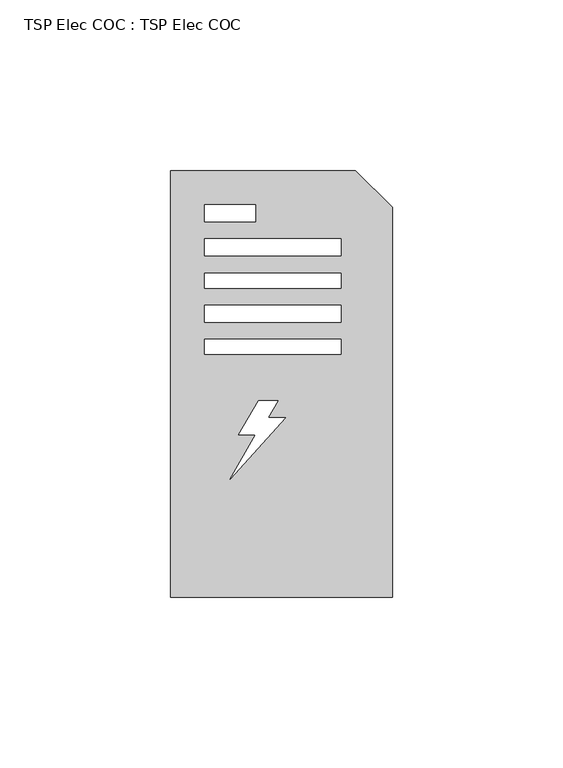
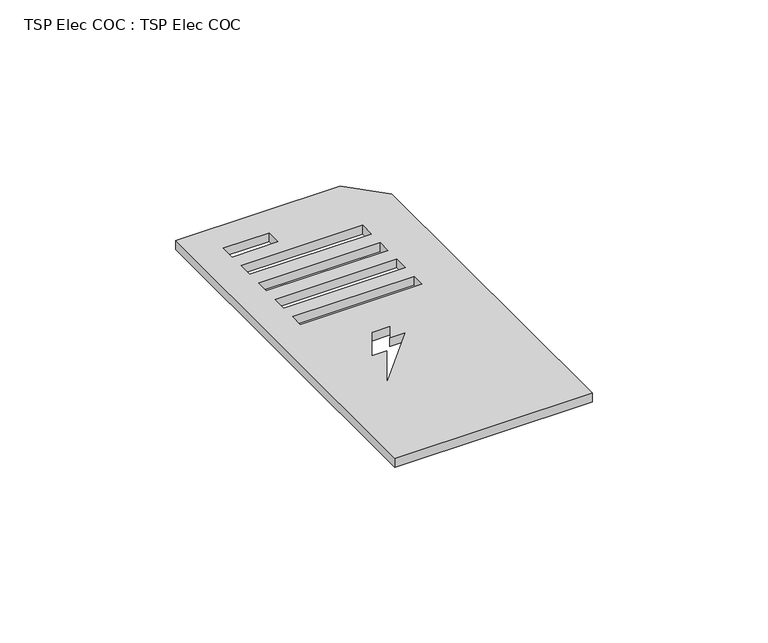
"""IFC4 building model written with IfcOpenShell, lengths in millimetres: proxy geometry, TSP Elec COC : TSP Elec COC."""

import ifcopenshell
import ifcopenshell.guid

model = None  # the IFC model being written
_history = None  # IfcOwnerHistory: only IFC2X3 demands one
_inside = {}  # id of a spatial element -> (the spatial element, [elements in it])
_under = {}  # id of a project, library or spatial element -> (it, [spatial elements below it])
_declared = {}  # id of a project -> (the project, [libraries it declares])
_typed = {}  # id of a type object -> (the type object, [elements of that type])
_made_of = {}  # id of a material, layer set ... -> (it, [elements and type objects made of it])


def new_model(schema):
    """Start an empty IFC model of exactly this schema.

    Asked for "IFC4X3", IfcOpenShell would pick the latest addendum, in which some entities
    have other attributes; the version numbers below select the first issue.
    IFC2X3 requires an IfcOwnerHistory on every rooted entity: one is made here for all.
    """
    global model, _history
    if schema == "IFC4X3":
        model = ifcopenshell.file(schema_version=(4, 3, 0, 0))
    else:
        model = ifcopenshell.file(schema=schema)
    _inside.clear()
    _under.clear()
    _declared.clear()
    _typed.clear()
    _made_of.clear()
    _history = None
    if model.schema == "IFC2X3":
        org = make("IfcOrganization", Name="unknown")
        user = make(
            "IfcPersonAndOrganization",
            ThePerson=make("IfcPerson", FamilyName="unknown"),
            TheOrganization=org,
        )
        app = make(
            "IfcApplication",
            ApplicationDeveloper=org,
            Version="unknown",
            ApplicationFullName="unknown",
            ApplicationIdentifier="unknown",
        )
        _history = make(
            "IfcOwnerHistory",
            OwningUser=user,
            OwningApplication=app,
            ChangeAction="ADDED",
            CreationDate=0,
        )
    return model


def make(cls, **values):
    """One entity of the class cls with the attributes given. An attribute that is None is left unset."""
    return model.create_entity(
        cls, **{name: value for name, value in values.items() if value is not None}
    )


def rooted(cls, **values):
    """An entity with a GlobalId (a new one), such as an element, a storey or a relation."""
    return make(cls, GlobalId=ifcopenshell.guid.new(), OwnerHistory=_history, **values)


def si_unit(unit_type, name, prefix=None):
    """IfcSIUnit, for example si_unit("LENGTHUNIT", "METRE", prefix="MILLI")."""
    return make("IfcSIUnit", UnitType=unit_type, Prefix=prefix, Name=name)


def assignment(units):
    """IfcUnitAssignment: the units of a project."""
    return None if units is None else make("IfcUnitAssignment", Units=units)


def point(xyz):
    """IfcCartesianPoint."""
    return None if xyz is None else make("IfcCartesianPoint", Coordinates=xyz)


def direction(xyz):
    """IfcDirection."""
    return None if xyz is None else make("IfcDirection", DirectionRatios=xyz)


def frame(location, z_axis=None, x_axis=None):
    """IfcAxis2Placement3D, a coordinate frame: its origin and axes. An axis left out is left unset."""
    return make(
        "IfcAxis2Placement3D",
        Location=point(location),
        Axis=direction(z_axis),
        RefDirection=direction(x_axis),
    )


def origin():
    """The frame at (0, 0, 0) with its axes left unset."""
    return frame((0.0, 0.0, 0.0))


def origin_with_axes():
    """The frame at (0, 0, 0) with the z axis (0, 0, 1) and the x axis (1, 0, 0) written out."""
    return frame((0.0, 0.0, 0.0), z_axis=(0.0, 0.0, 1.0), x_axis=(1.0, 0.0, 0.0))


def place(relative_to, where):
    """IfcLocalPlacement: puts the frame where relative to a parent placement (None: the world)."""
    return make(
        "IfcLocalPlacement", PlacementRelTo=relative_to, RelativePlacement=where
    )


def context(
    kind, dimensions, precision=None, world=None, true_north=None, identifier=None
):
    """IfcGeometricRepresentationContext, for example the 3D "Model" context."""
    return make(
        "IfcGeometricRepresentationContext",
        ContextIdentifier=identifier,
        ContextType=kind,
        CoordinateSpaceDimension=dimensions,
        Precision=precision,
        WorldCoordinateSystem=world,
        TrueNorth=true_north,
    )


def project(units=None, contexts=None):
    """IfcProject with its units and contexts."""
    return rooted(
        "IfcProject",
        Name="project",
        RepresentationContexts=contexts,
        UnitsInContext=assignment(units),
    )


def spatial(cls, under=None, at=None, **own):
    """A site, building, storey or space (cls), placed at a placement, below another one or the project."""
    s = rooted(cls, ObjectPlacement=at, **own)
    if under is not None:
        _under.setdefault(under.id(), (under, []))[1].append(s)
    return s


def polyline(points):
    """IfcPolyline through the points."""
    return make("IfcPolyline", Points=[point(p) for p in points])


def outline(outer, holes=None, kind="AREA"):
    """IfcArbitraryClosedProfileDef: a profile drawn as a closed curve; with holes, ...WithVoids."""
    if holes is None:
        return make("IfcArbitraryClosedProfileDef", ProfileType=kind, OuterCurve=outer)
    return make(
        "IfcArbitraryProfileDefWithVoids",
        ProfileType=kind,
        OuterCurve=outer,
        InnerCurves=holes,
    )


def extrude(swept, where, along, depth):
    """IfcExtrudedAreaSolid: the profile swept, set in the frame where, extruded along a direction by depth."""
    return make(
        "IfcExtrudedAreaSolid",
        SweptArea=swept,
        Position=where,
        ExtrudedDirection=direction(along),
        Depth=depth,
    )


def shape(context_of_items, identifier, shape_type, items):
    """IfcShapeRepresentation: the items that make up one representation, for example the "Body"."""
    return make(
        "IfcShapeRepresentation",
        ContextOfItems=context_of_items,
        RepresentationIdentifier=identifier,
        RepresentationType=shape_type,
        Items=items,
    )


def source(mapping_origin, context_of_items, identifier, shape_type, items):
    """IfcRepresentationMap: a shape defined once, which mapped items show again and again."""
    return make(
        "IfcRepresentationMap",
        MappingOrigin=mapping_origin,
        MappedRepresentation=shape(context_of_items, identifier, shape_type, items),
    )


def transform(
    local_origin,
    x_axis=None,
    y_axis=None,
    z_axis=None,
    scale=None,
    scale2=None,
    scale3=None,
    uniform=True,
):
    """IfcCartesianTransformationOperator3D, or its non-uniform kind. x_axis, y_axis, z_axis: its Axis1, 2, 3."""
    if uniform:
        return make(
            "IfcCartesianTransformationOperator3D",
            Axis1=direction(x_axis),
            Axis2=direction(y_axis),
            LocalOrigin=point(local_origin),
            Scale=scale,
            Axis3=direction(z_axis),
        )
    return make(
        "IfcCartesianTransformationOperator3DnonUniform",
        Axis1=direction(x_axis),
        Axis2=direction(y_axis),
        LocalOrigin=point(local_origin),
        Scale=scale,
        Axis3=direction(z_axis),
        Scale2=scale2,
        Scale3=scale3,
    )


def mapped(mapping_source, mapping_target):
    """IfcMappedItem: shows the shape of a source again, moved by a transform."""
    return make(
        "IfcMappedItem", MappingSource=mapping_source, MappingTarget=mapping_target
    )


def made_of(thing, what):
    """Note that an element or type object is made of a material, layer set ...; save() writes the relation."""
    if what is not None:
        _made_of.setdefault(what.id(), (what, []))[1].append(thing)
    return thing


def element(
    cls,
    number,
    at=None,
    inside=None,
    cuts=None,
    type_object=None,
    material=None,
    context=None,
    identifier="Body",
    shape_type=None,
    held_by="IfcProductDefinitionShape",
    body=None,
    shapes=None,
    **own,
):
    """One element of the class cls, such as IfcWall. Its Tag is "e" and its number.

    at: its placement. inside: the storey or other place that contains it. cuts: it is an
    opening in that element (IfcRelVoidsElement). A single representation is given by context,
    identifier, shape_type and body (its items); several are given by shapes. held_by: the class
    of the entity that holds the representations. save() writes the other relations.
    """
    e = rooted(cls, Tag="e%d" % number, ObjectPlacement=at, **own)
    if body is not None:
        shapes = [shape(context, identifier, shape_type, body)]
    if shapes is not None:
        e.Representation = make(held_by, Representations=shapes)
    if inside is not None:
        _inside.setdefault(inside.id(), (inside, []))[1].append(e)
    if cuts is not None:
        rooted(
            "IfcRelVoidsElement", RelatingBuildingElement=cuts, RelatedOpeningElement=e
        )
    if type_object is not None:
        _typed.setdefault(type_object.id(), (type_object, []))[1].append(e)
    return made_of(e, material)


def aggregate(whole, parts):
    """IfcRelAggregates: a whole, such as a stair, and the parts it consists of."""
    return rooted("IfcRelAggregates", RelatingObject=whole, RelatedObjects=parts)


def save(model, path):
    """Write the relations noted so far, then the file.

    IfcRelAggregates (storeys below a building ...), IfcRelContainedInSpatialStructure (elements
    in a storey), IfcRelDefinesByType, IfcRelAssociatesMaterial and IfcRelDeclares: one each for
    every whole, place, type object, material and project.
    """
    for whole, parts in _under.values():
        aggregate(whole, parts)
    for where, things in _inside.values():
        rooted(
            "IfcRelContainedInSpatialStructure",
            RelatedElements=things,
            RelatingStructure=where,
        )
    for kind, things in _typed.values():
        rooted("IfcRelDefinesByType", RelatedObjects=things, RelatingType=kind)
    for what, things in _made_of.values():
        rooted("IfcRelAssociatesMaterial", RelatedObjects=things, RelatingMaterial=what)
    for by, libraries in _declared.values():
        rooted("IfcRelDeclares", RelatingContext=by, RelatedDefinitions=libraries)
    model.write(path)


def tsp_elec_coc_tsp_elec_coc_e81222bd(model_context):
    return source(origin(), model_context, "Body", "SweptSolid", [
        extrude(outline(polyline([(-65.0, 60.0), (-10.7447385, 60.0), (0.0, 49.2552615), (0.0, -65.0), (-65.0, -65.0), (-65.0, 60.0)]), holes=[polyline([(-40.0, 50.0), (-55.0, 50.0), (-55.0, 45.0), (-40.0, 45.0), (-40.0, 50.0)]), polyline([(-15.0, 40.0), (-55.0, 40.0), (-55.0, 35.0), (-15.0, 35.0), (-15.0, 40.0)]), polyline([(-15.0, 30.0), (-55.0, 30.0), (-55.0, 25.6203938), (-15.0, 25.6203938), (-15.0, 30.0)]), polyline([(-15.0, 20.6203938), (-55.0, 20.6203938), (-55.0, 15.6203938), (-15.0, 15.6203938), (-15.0, 20.6203938)]), polyline([(-15.0, 10.6203938), (-55.0, 10.6203938), (-55.0, 6.2407877), (-15.0, 6.2407877), (-15.0, 10.6203938)]), polyline([(-33.4529946, -7.4194663), (-39.2264973, -7.4194663), (-45.0, -17.4194663), (-40.0, -17.4194663), (-47.5, -30.4098474), (-31.339746, -12.4194663), (-36.339746, -12.4194663), (-33.4529946, -7.4194663)])]), origin_with_axes(), (0.0, 0.0, 1.0), 3.0),
    ])


if __name__ == "__main__":
    model = new_model("IFC4")
    model_context = context("Model", 3, world=origin())
    ifc_project = project(units=[si_unit("LENGTHUNIT", "METRE", prefix="MILLI")], contexts=[model_context])
    site = spatial("IfcSite", under=ifc_project)
    building = spatial("IfcBuilding", under=site)
    placement = place(None, origin())
    tsp_elec_coc_tsp_elec_coc_shape = tsp_elec_coc_tsp_elec_coc_e81222bd(model_context)
    element("IfcBuildingElementProxy", 1, Name="TSP Elec COC : TSP Elec COC", ObjectType="TSP Elec COC : TSP Elec COC", at=placement, inside=building, context=model_context, shape_type="MappedRepresentation", body=[
        mapped(tsp_elec_coc_tsp_elec_coc_shape, transform((0.0, 0.0, 0.0), x_axis=(1.0, 0.0, 0.0), y_axis=(0.0, 1.0, 0.0), z_axis=(0.0, 0.0, 1.0))),
    ])
    save(model, "model.ifc")

# Revit data of these elements
# Type "TSP Elec COC : TSP Elec COC"
#   Model = "TSP_ELECCERC"
#   Default Elevation = 0
# Element 1 (IfcBuildingElementProxy, "TSP Elec COC : TSP Elec COC")
#   Materials on its faces: "Plastic, Opaque Black"
# Materials
#   "Plastic, Opaque Black": class "Plastic", colour RGB 0 0 0, transparency 0.7, Description = "Plastic, generic, opaque black", Cost = 0
